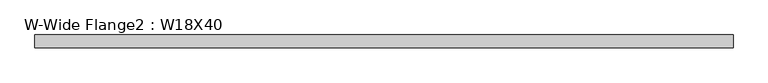
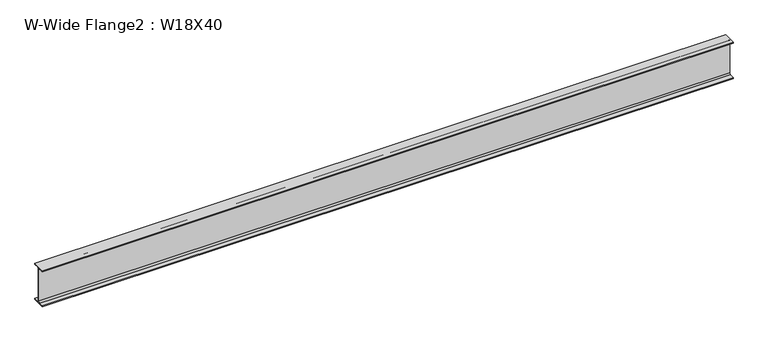
"""IFC4 building model written with IfcOpenShell, lengths in millimetres: beam geometry, W-Wide Flange2 : W18X40."""

from ifc_helpers import new_model, si_unit, point, frame, frame_2d, origin, place, context, project, spatial, polyline, circle_curve, trimmed, segment, composite_curve, outline, extrude, source, transform, mapped, element, save


def w_wide_flange2_w18x40_41391f11(model_context):
    return source(origin(), model_context, "Body", "SweptSolid", [
        extrude(outline(composite_curve([segment(polyline([(76.454, -213.995), (76.454, -227.33), (-76.454, -227.33), (-76.454, -213.995), (-20.828, -213.995)]), True, "CONTINUOUS"), segment(trimmed(circle_curve(frame_2d((-20.828, -197.1675)), 16.8275), [point((-20.828, -213.995))], [point((-4.0005, -197.1675))], True, "CARTESIAN"), True, "CONTINUOUS"), segment(polyline([(-4.0005, -197.1675), (-4.0005, 197.1675)]), True, "CONTINUOUS"), segment(trimmed(circle_curve(frame_2d((-20.828, 197.1675)), 16.8275), [point((-4.0005, 197.1675))], [point((-20.828, 213.995))], True, "CARTESIAN"), True, "CONTINUOUS"), segment(polyline([(-20.828, 213.995), (-76.454, 213.995), (-76.454, 227.33), (76.454, 227.33), (76.454, 213.995), (20.828, 213.995)]), True, "CONTINUOUS"), segment(trimmed(circle_curve(frame_2d((20.828, 197.1675)), 16.8275), [point((20.828, 213.995))], [point((4.0005, 197.1675))], True, "CARTESIAN"), True, "CONTINUOUS"), segment(polyline([(4.0005, 197.1675), (4.0005, -197.1675)]), True, "CONTINUOUS"), segment(trimmed(circle_curve(frame_2d((20.828, -197.1675)), 16.8275), [point((4.0005, -197.1675))], [point((20.828, -213.995))], True, "CARTESIAN"), True, "CONTINUOUS"), segment(polyline([(20.828, -213.995), (76.454, -213.995)]), True, "CONTINUOUS")], self_intersect=False)), frame((-4095.353125, 0.0, 0.0), z_axis=(1.0, 0.0, 0.0), x_axis=(0.0, 1.0, 0.0)), (0.0, 0.0, 1.0), 8190.70625),
    ])


if __name__ == "__main__":
    model = new_model("IFC4")
    model_context = context("Model", 3, world=origin())
    ifc_project = project(units=[si_unit("LENGTHUNIT", "METRE", prefix="MILLI")], contexts=[model_context])
    site = spatial("IfcSite", under=ifc_project)
    building = spatial("IfcBuilding", under=site)
    placement = place(None, origin())
    w_wide_flange2_w18x40_shape = w_wide_flange2_w18x40_41391f11(model_context)
    element("IfcBeam", 1, ObjectType="W-Wide Flange2 : W18X40", at=placement, inside=building, context=model_context, shape_type="MappedRepresentation", body=[
        mapped(w_wide_flange2_w18x40_shape, transform((0.0, 0.0, 0.0), x_axis=(1.0, 0.0, 0.0), y_axis=(0.0, 1.0, 0.0), z_axis=(0.0, 0.0, 1.0))),
    ])
    save(model, "model.ifc")

# Revit data of these elements
# Type "W-Wide Flange2 : W18X40"
#   Assembly Code = "B10"
#   W = 40
#   Length [instance default] = 5' - 0"
#   bf = 0' - 6.02"
#   d = 1' - 5.9"
#   k = 0' - 1 3/16"
#   k2 = 0' - 0.6625"
#   tf = 0' - 0.525"
#   tw = 0' - 0.315"
#   A = 0.0819444 SF
#   Structural Material [instance default] = Steel ASTM A992
# Element 1 (IfcBeam, "W-Wide Flange2 : W18X40")
#   Materials on its faces: "Steel ASTM A992"
# Materials
#   "Steel ASTM A992": class "Metal", colour RGB 199 199 199, transparency 0, Description = "Structural steel 50ksi", Cost = 0
